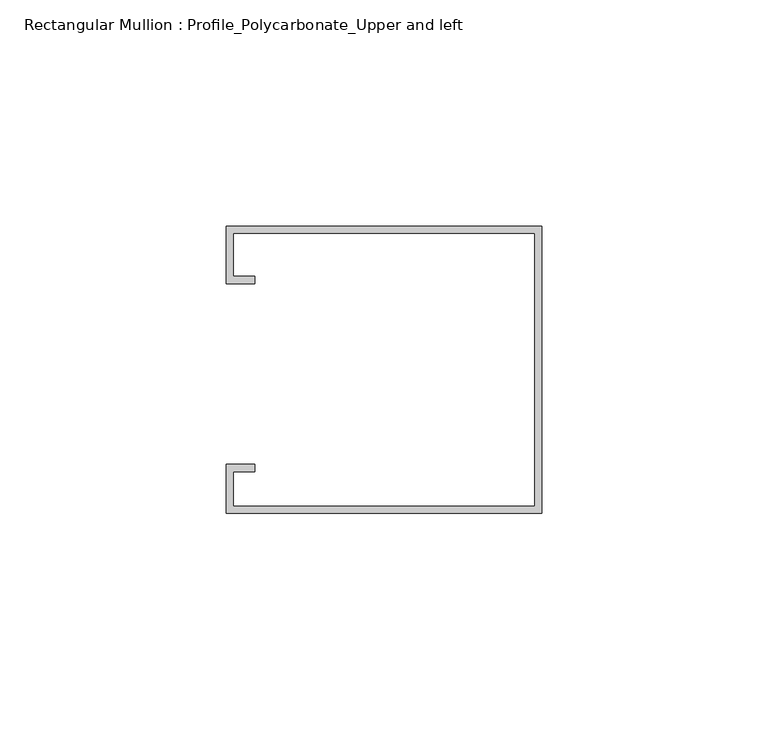
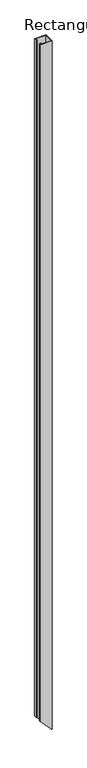
"""IFC4 building model written with IfcOpenShell, lengths in millimetres: member geometry, Rectangular Mullion : Profile_Polycarbonate_Upper and left."""

import ifcopenshell
import ifcopenshell.guid

model = None  # the IFC model being written
_history = None  # IfcOwnerHistory: only IFC2X3 demands one
_inside = {}  # id of a spatial element -> (the spatial element, [elements in it])
_under = {}  # id of a project, library or spatial element -> (it, [spatial elements below it])
_declared = {}  # id of a project -> (the project, [libraries it declares])
_typed = {}  # id of a type object -> (the type object, [elements of that type])
_made_of = {}  # id of a material, layer set ... -> (it, [elements and type objects made of it])


def new_model(schema):
    """Start an empty IFC model of exactly this schema.

    Asked for "IFC4X3", IfcOpenShell would pick the latest addendum, in which some entities
    have other attributes; the version numbers below select the first issue.
    IFC2X3 requires an IfcOwnerHistory on every rooted entity: one is made here for all.
    """
    global model, _history
    if schema == "IFC4X3":
        model = ifcopenshell.file(schema_version=(4, 3, 0, 0))
    else:
        model = ifcopenshell.file(schema=schema)
    _inside.clear()
    _under.clear()
    _declared.clear()
    _typed.clear()
    _made_of.clear()
    _history = None
    if model.schema == "IFC2X3":
        org = make("IfcOrganization", Name="unknown")
        user = make(
            "IfcPersonAndOrganization",
            ThePerson=make("IfcPerson", FamilyName="unknown"),
            TheOrganization=org,
        )
        app = make(
            "IfcApplication",
            ApplicationDeveloper=org,
            Version="unknown",
            ApplicationFullName="unknown",
            ApplicationIdentifier="unknown",
        )
        _history = make(
            "IfcOwnerHistory",
            OwningUser=user,
            OwningApplication=app,
            ChangeAction="ADDED",
            CreationDate=0,
        )
    return model


def make(cls, **values):
    """One entity of the class cls with the attributes given. An attribute that is None is left unset."""
    return model.create_entity(
        cls, **{name: value for name, value in values.items() if value is not None}
    )


def rooted(cls, **values):
    """An entity with a GlobalId (a new one), such as an element, a storey or a relation."""
    return make(cls, GlobalId=ifcopenshell.guid.new(), OwnerHistory=_history, **values)


def si_unit(unit_type, name, prefix=None):
    """IfcSIUnit, for example si_unit("LENGTHUNIT", "METRE", prefix="MILLI")."""
    return make("IfcSIUnit", UnitType=unit_type, Prefix=prefix, Name=name)


def assignment(units):
    """IfcUnitAssignment: the units of a project."""
    return None if units is None else make("IfcUnitAssignment", Units=units)


def point(xyz):
    """IfcCartesianPoint."""
    return None if xyz is None else make("IfcCartesianPoint", Coordinates=xyz)


def direction(xyz):
    """IfcDirection."""
    return None if xyz is None else make("IfcDirection", DirectionRatios=xyz)


def frame(location, z_axis=None, x_axis=None):
    """IfcAxis2Placement3D, a coordinate frame: its origin and axes. An axis left out is left unset."""
    return make(
        "IfcAxis2Placement3D",
        Location=point(location),
        Axis=direction(z_axis),
        RefDirection=direction(x_axis),
    )


def origin():
    """The frame at (0, 0, 0) with its axes left unset."""
    return frame((0.0, 0.0, 0.0))


def place(relative_to, where):
    """IfcLocalPlacement: puts the frame where relative to a parent placement (None: the world)."""
    return make(
        "IfcLocalPlacement", PlacementRelTo=relative_to, RelativePlacement=where
    )


def context(
    kind, dimensions, precision=None, world=None, true_north=None, identifier=None
):
    """IfcGeometricRepresentationContext, for example the 3D "Model" context."""
    return make(
        "IfcGeometricRepresentationContext",
        ContextIdentifier=identifier,
        ContextType=kind,
        CoordinateSpaceDimension=dimensions,
        Precision=precision,
        WorldCoordinateSystem=world,
        TrueNorth=true_north,
    )


def project(units=None, contexts=None):
    """IfcProject with its units and contexts."""
    return rooted(
        "IfcProject",
        Name="project",
        RepresentationContexts=contexts,
        UnitsInContext=assignment(units),
    )


def spatial(cls, under=None, at=None, **own):
    """A site, building, storey or space (cls), placed at a placement, below another one or the project."""
    s = rooted(cls, ObjectPlacement=at, **own)
    if under is not None:
        _under.setdefault(under.id(), (under, []))[1].append(s)
    return s


def faces_of(points, faces, orient=None, outer=None):
    """IfcFace entities. A face is a list of loops; a loop is a list of indices into points, from 0.

    orient and outer hold one flag for each loop. By default every Orientation is true, the
    first loop of a face is its IfcFaceOuterBound and the others are IfcFaceBound.
    """
    made = []
    for i, loops in enumerate(faces):
        bounds = []
        for j, loop in enumerate(loops):
            is_outer = j == 0 if outer is None else outer[i][j]
            bounds.append(
                make(
                    "IfcFaceOuterBound" if is_outer else "IfcFaceBound",
                    Bound=make("IfcPolyLoop", Polygon=[points[k] for k in loop]),
                    Orientation=True if orient is None else orient[i][j],
                )
            )
        made.append(make("IfcFace", Bounds=bounds))
    return made


def faceted_brep(points, faces, orient=None, outer=None, voids=None):
    """IfcFacetedBrep: a solid bounded by flat faces; with voids (closed shells), ...WithVoids."""
    shared = [point(p) for p in points]
    hull = make("IfcClosedShell", CfsFaces=faces_of(shared, faces, orient, outer))
    if voids is None:
        return make("IfcFacetedBrep", Outer=hull)
    return make(
        "IfcFacetedBrepWithVoids",
        Outer=hull,
        Voids=[
            make(cls, CfsFaces=faces_of(shared, fs, o, b)) for cls, fs, o, b in voids
        ],
    )


def shape(context_of_items, identifier, shape_type, items):
    """IfcShapeRepresentation: the items that make up one representation, for example the "Body"."""
    return make(
        "IfcShapeRepresentation",
        ContextOfItems=context_of_items,
        RepresentationIdentifier=identifier,
        RepresentationType=shape_type,
        Items=items,
    )


def source(mapping_origin, context_of_items, identifier, shape_type, items):
    """IfcRepresentationMap: a shape defined once, which mapped items show again and again."""
    return make(
        "IfcRepresentationMap",
        MappingOrigin=mapping_origin,
        MappedRepresentation=shape(context_of_items, identifier, shape_type, items),
    )


def transform(
    local_origin,
    x_axis=None,
    y_axis=None,
    z_axis=None,
    scale=None,
    scale2=None,
    scale3=None,
    uniform=True,
):
    """IfcCartesianTransformationOperator3D, or its non-uniform kind. x_axis, y_axis, z_axis: its Axis1, 2, 3."""
    if uniform:
        return make(
            "IfcCartesianTransformationOperator3D",
            Axis1=direction(x_axis),
            Axis2=direction(y_axis),
            LocalOrigin=point(local_origin),
            Scale=scale,
            Axis3=direction(z_axis),
        )
    return make(
        "IfcCartesianTransformationOperator3DnonUniform",
        Axis1=direction(x_axis),
        Axis2=direction(y_axis),
        LocalOrigin=point(local_origin),
        Scale=scale,
        Axis3=direction(z_axis),
        Scale2=scale2,
        Scale3=scale3,
    )


def mapped(mapping_source, mapping_target):
    """IfcMappedItem: shows the shape of a source again, moved by a transform."""
    return make(
        "IfcMappedItem", MappingSource=mapping_source, MappingTarget=mapping_target
    )


def made_of(thing, what):
    """Note that an element or type object is made of a material, layer set ...; save() writes the relation."""
    if what is not None:
        _made_of.setdefault(what.id(), (what, []))[1].append(thing)
    return thing


def element(
    cls,
    number,
    at=None,
    inside=None,
    cuts=None,
    type_object=None,
    material=None,
    context=None,
    identifier="Body",
    shape_type=None,
    held_by="IfcProductDefinitionShape",
    body=None,
    shapes=None,
    **own,
):
    """One element of the class cls, such as IfcWall. Its Tag is "e" and its number.

    at: its placement. inside: the storey or other place that contains it. cuts: it is an
    opening in that element (IfcRelVoidsElement). A single representation is given by context,
    identifier, shape_type and body (its items); several are given by shapes. held_by: the class
    of the entity that holds the representations. save() writes the other relations.
    """
    e = rooted(cls, Tag="e%d" % number, ObjectPlacement=at, **own)
    if body is not None:
        shapes = [shape(context, identifier, shape_type, body)]
    if shapes is not None:
        e.Representation = make(held_by, Representations=shapes)
    if inside is not None:
        _inside.setdefault(inside.id(), (inside, []))[1].append(e)
    if cuts is not None:
        rooted(
            "IfcRelVoidsElement", RelatingBuildingElement=cuts, RelatedOpeningElement=e
        )
    if type_object is not None:
        _typed.setdefault(type_object.id(), (type_object, []))[1].append(e)
    return made_of(e, material)


def aggregate(whole, parts):
    """IfcRelAggregates: a whole, such as a stair, and the parts it consists of."""
    return rooted("IfcRelAggregates", RelatingObject=whole, RelatedObjects=parts)


def save(model, path):
    """Write the relations noted so far, then the file.

    IfcRelAggregates (storeys below a building ...), IfcRelContainedInSpatialStructure (elements
    in a storey), IfcRelDefinesByType, IfcRelAssociatesMaterial and IfcRelDeclares: one each for
    every whole, place, type object, material and project.
    """
    for whole, parts in _under.values():
        aggregate(whole, parts)
    for where, things in _inside.values():
        rooted(
            "IfcRelContainedInSpatialStructure",
            RelatedElements=things,
            RelatingStructure=where,
        )
    for kind, things in _typed.values():
        rooted("IfcRelDefinesByType", RelatedObjects=things, RelatingType=kind)
    for what, things in _made_of.values():
        rooted("IfcRelAssociatesMaterial", RelatedObjects=things, RelatingMaterial=what)
    for by, libraries in _declared.values():
        rooted("IfcRelDeclares", RelatingContext=by, RelatedDefinitions=libraries)
    model.write(path)


def rectangular_mullion_profile_polycarbonate_upper_and_left_05964faa(model_context):
    return source(origin(), model_context, "Body", "Brep", [
        faceted_brep([(0.0, 32.7, 0.0), (-69.85, 32.7, 0.0), (-69.85, 20.0, 0.0), (-63.5, 20.0, 0.0), (-63.5, 21.5875, 0.0), (-68.2625, 21.5875, 0.0), (-68.2625, 31.1125, 0.0), (-1.5875, 31.1125, 0.0), (-1.5875, -29.2125, 0.0), (-68.2625, -29.2125, 0.0), (-68.2625, -21.5875, 0.0), (-63.5, -21.5875, 0.0), (-63.5, -20.0, 0.0), (-69.85, -20.0, 0.0), (-69.85, -30.8, 0.0), (0.0, -30.8, 0.0), (0.0, 32.7, -4472.3181431), (-69.85, 32.7, -4399.4971191), (-69.85, 20.0, -4399.4971191), (-63.5, 20.0, -4406.1172122), (-63.5, 21.5875, -4406.1172122), (-68.2625, 21.5875, -4401.1521423), (-68.2625, 31.1125, -4401.1521423), (-1.5875, 31.1125, -4470.6631198), (-1.5875, -29.2125, -4470.6631198), (-68.2625, -29.2125, -4401.1521423), (-68.2625, -21.5875, -4401.1521423), (-63.5, -21.5875, -4406.1172122), (-63.5, -20.0, -4406.1172122), (-69.85, -20.0, -4399.4971191), (-69.85, -30.8, -4399.4971191), (0.0, -30.8, -4472.3181431)], [[[0, 1, 2, 3, 4, 5, 6, 7, 8, 9, 10, 11, 12, 13, 14, 15]], [[1, 0, 16, 17]], [[2, 1, 17, 18]], [[3, 2, 18, 19]], [[4, 3, 19, 20]], [[5, 4, 20, 21]], [[6, 5, 21, 22]], [[7, 6, 22, 23]], [[8, 7, 23, 24]], [[9, 8, 24, 25]], [[10, 9, 25, 26]], [[11, 10, 26, 27]], [[12, 11, 27, 28]], [[13, 12, 28, 29]], [[14, 13, 29, 30]], [[15, 14, 30, 31]], [[0, 15, 31, 16]], [[16, 31, 30, 29, 28, 27, 26, 25, 24, 23, 22, 21, 20, 19, 18, 17]]]),
    ])


if __name__ == "__main__":
    model = new_model("IFC4")
    model_context = context("Model", 3, world=origin())
    ifc_project = project(units=[si_unit("LENGTHUNIT", "METRE", prefix="MILLI")], contexts=[model_context])
    site = spatial("IfcSite", under=ifc_project)
    building = spatial("IfcBuilding", under=site)
    placement = place(None, origin())
    rectangular_mullion_profile_polycarbonate_upper_and_left_shape = rectangular_mullion_profile_polycarbonate_upper_and_left_05964faa(model_context)
    element("IfcMember", 1, ObjectType="Rectangular Mullion : Profile_Polycarbonate_Upper and left", at=placement, inside=building, context=model_context, shape_type="MappedRepresentation", body=[
        mapped(rectangular_mullion_profile_polycarbonate_upper_and_left_shape, transform((0.0, 0.0, 0.0), x_axis=(1.0, 0.0, 0.0), y_axis=(0.0, 1.0, 0.0), z_axis=(0.0, 0.0, 1.0))),
    ])
    save(model, "model.ifc")

# Revit data of these elements
# Type "Rectangular Mullion : Profile_Polycarbonate_Upper and left"
#   built-in parameter 1007322 = 0.208333 (stored number, unit not read)
#   built-in parameter 1007321 = 0.00520833 (stored number, unit not read)
#   built-in parameter 1007320 = 0 (stored number, unit not read)
